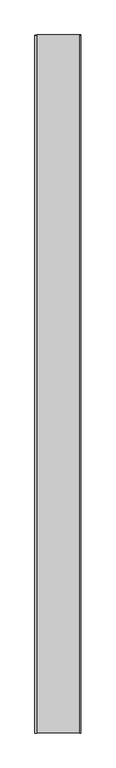
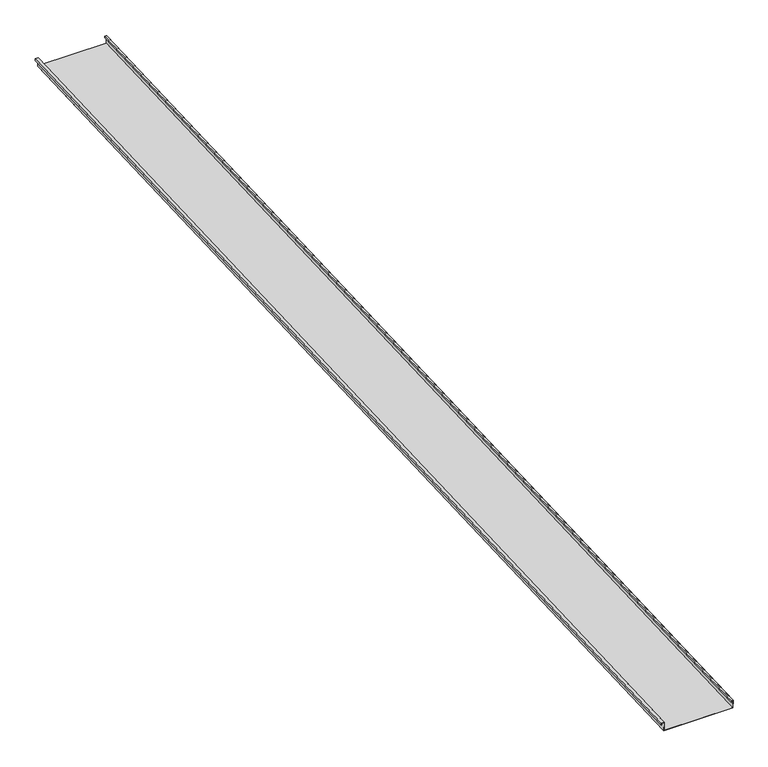
"""IFC4 building model written with IfcOpenShell, lengths in millimetres: proxy geometry, Generic Models 2:Generic Models 2:310765:Generic Models 2:310765 : Generic Models 2:Generic Models 2:310765:110 : Generic Models 2:Generic Models 2:310765:Generic Models 2:310765 : Generic Models 2:Generic Models 2:310765:300385."""

from ifc_helpers import new_model, si_unit, frame, origin, place, context, project, spatial, polyline, outline, extrude, source, transform, mapped, element, save


def generic_models_9905db8b(model_context):
    return source(origin(), model_context, "Body", "SweptSolid", [
        extrude(outline(polyline([(1.5875, 0.0), (1.5875, 50.8), (407.9875, 50.8), (407.9875, 1.5875), (396.875, 1.5875), (396.875, 11.1125), (398.4625, 11.1125), (398.4625, 3.175), (406.4, 3.175), (406.4, 49.2125), (3.175, 49.2125), (3.175, -1.5874999), (-14.2875, -1.5874999), (-14.2875, 9.525), (-12.7, 9.525), (-12.7, 0.0), (1.5875, 0.0)])), frame((609059.8429739, -581354.4345603, 3902.6697972), z_axis=(0.0, 0.9991330730923568, 0.041630544712067834), x_axis=(1.0, 0.0, 0.0)), (0.0, 0.0, 1.0), 6400.8),
    ])


if __name__ == "__main__":
    model = new_model("IFC4")
    model_context = context("Model", 3, world=origin())
    ifc_project = project(units=[si_unit("LENGTHUNIT", "METRE", prefix="MILLI")], contexts=[model_context])
    site = spatial("IfcSite", under=ifc_project)
    building = spatial("IfcBuilding", under=site)
    placement = place(None, origin())
    generic_models_shape = generic_models_9905db8b(model_context)
    element("IfcBuildingElementProxy", 1, Name="Generic Models 2:Generic Models 2:310765:Generic Models 2:310765 : Generic Models 2:Generic Models 2:310765:110 : Generic Models 2:Generic Models 2:310765:Generic Models 2:310765 : Generic Models 2:Generic Models 2:310765:300385", ObjectType="Generic Models 2:Generic Models 2:310765:Generic Models 2:310765 : Generic Models 2:Generic Models 2:310765:110 : Generic Models 2:Generic Models 2:310765:Generic Models 2:310765 : Generic Models 2:Generic Models 2:310765:300385", at=placement, inside=building, context=model_context, shape_type="MappedRepresentation", body=[
        mapped(generic_models_shape, transform((0.0, 0.0, 0.0), x_axis=(1.0, 0.0, 0.0), y_axis=(0.0, 1.0, 0.0), z_axis=(0.0, 0.0, 1.0))),
    ])
    save(model, "model.ifc")

# Revit data of these elements
# Type "Generic Models 2:Generic Models 2:310765:Generic Models 2:310765 : Generic Models 2:Generic Models 2:310765:110 : Generic Models 2:Generic Models 2:310765:Generic Models 2:310765 : Generic Models 2:Generic Models 2:310765:300385"
#   NameOverride = "Generic Models 2:Generic Models 2:310765:Generic Models 2:310765 : Generic Models 2:Generic Models 2:310765:300385"
#   ObjectTypeOverride = "Generic Models 2:310765 : Generic Models 2:Generic Models 2:310765"
#   Reference = "Generic Models 2"
#   Tag = "300385"
# Element 1 (IfcBuildingElementProxy, "Generic Models 2:Generic Models 2:310765:Generic Models 2:310765 : Generic Models 2:Generic Models 2:310765:110 : Generic Models 2:Generic Models 2:310765:Generic Models 2:310765 : Generic Models 2:Generic Models 2:310765:300385")
#   Materials on its faces: "THERMAL BROKEN ALUMINUM STOREFRONT FOR POLYCARBONATE"
# Materials
#   "THERMAL BROKEN ALUMINUM STOREFRONT FOR POLYCARBONATE": class "Unassigned", colour RGB 244 244 244, transparency 0, Keynote = "M07611300.01", Cost = 0
